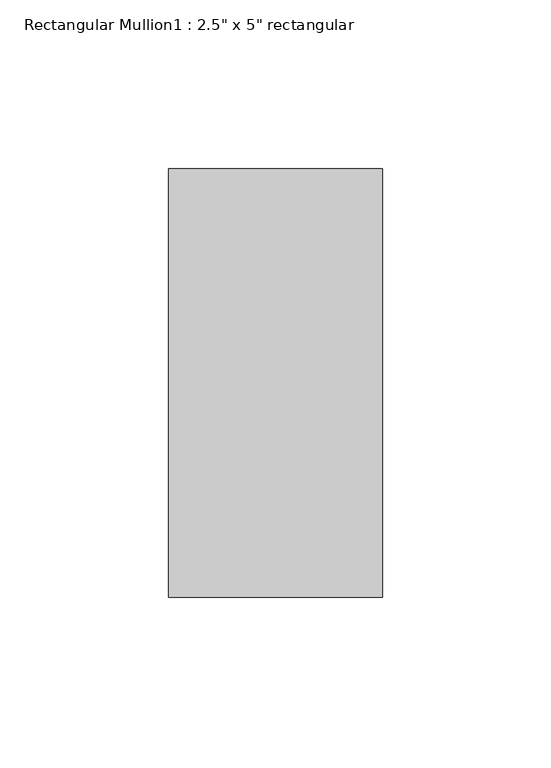
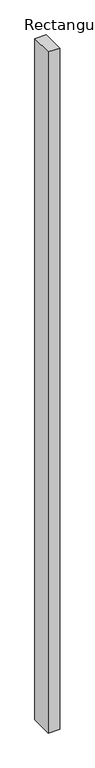
"""IFC4 building model written with IfcOpenShell, lengths in millimetres: member geometry."""

from ifc_helpers import new_model, si_unit, frame, origin, place, context, project, spatial, polyline, outline, extrude, source, transform, mapped, element, save


def member_5d333a65(model_context):
    return source(origin(), model_context, "Body", "SweptSolid", [
        extrude(outline(polyline([(0.0, 63.5), (0.0, -63.5), (-63.5, -63.5), (-63.5, 63.5), (0.0, 63.5)])), frame((0.0, 0.0, -3971.7835741), z_axis=(0.0, 0.0, 1.0), x_axis=(1.0, 0.0, 0.0)), (0.0, 0.0, 1.0), 3971.7835741),
    ])


if __name__ == "__main__":
    model = new_model("IFC4")
    model_context = context("Model", 3, world=origin())
    ifc_project = project(units=[si_unit("LENGTHUNIT", "METRE", prefix="MILLI")], contexts=[model_context])
    site = spatial("IfcSite", under=ifc_project)
    building = spatial("IfcBuilding", under=site)
    placement = place(None, origin())
    member_shape = member_5d333a65(model_context)
    element("IfcMember", 1, ObjectType="Rectangular Mullion1 : 2.5\" x 5\" rectangular", at=placement, inside=building, context=model_context, shape_type="MappedRepresentation", body=[
        mapped(member_shape, transform((0.0, 0.0, 0.0), x_axis=(1.0, 0.0, 0.0), y_axis=(0.0, 1.0, 0.0), z_axis=(0.0, 0.0, 1.0))),
    ])
    save(model, "model.ifc")

# Revit data of these elements
# Type "Rectangular Mullion1 : 2.5\" x 5\" rectangular"
#   built-in parameter 1007304 = 0.416667 (stored number, unit not read)
#   built-in parameter 1007301 = 0.104167 (stored number, unit not read)
#   built-in parameter 1007300 = 0.104167 (stored number, unit not read)
# Element 1 (IfcMember, "Rectangular Mullion1 : 2.5\" x 5\" rectangular")
#   Materials on its faces: "support-frame"
# Materials
#   "support-frame": class "Unassigned", colour RGB 233 233 233, transparency 0, Cost = 0
